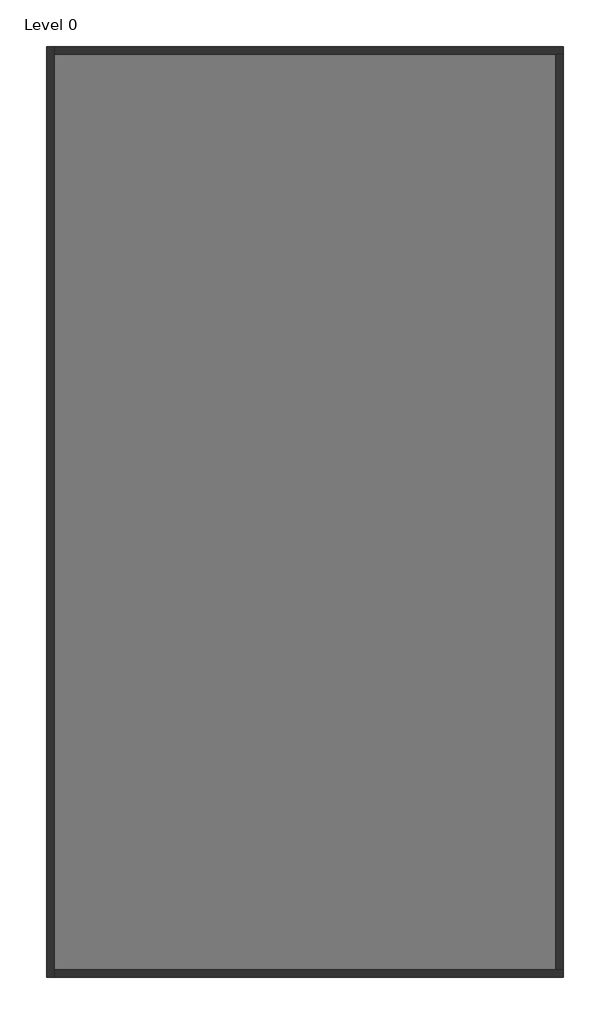
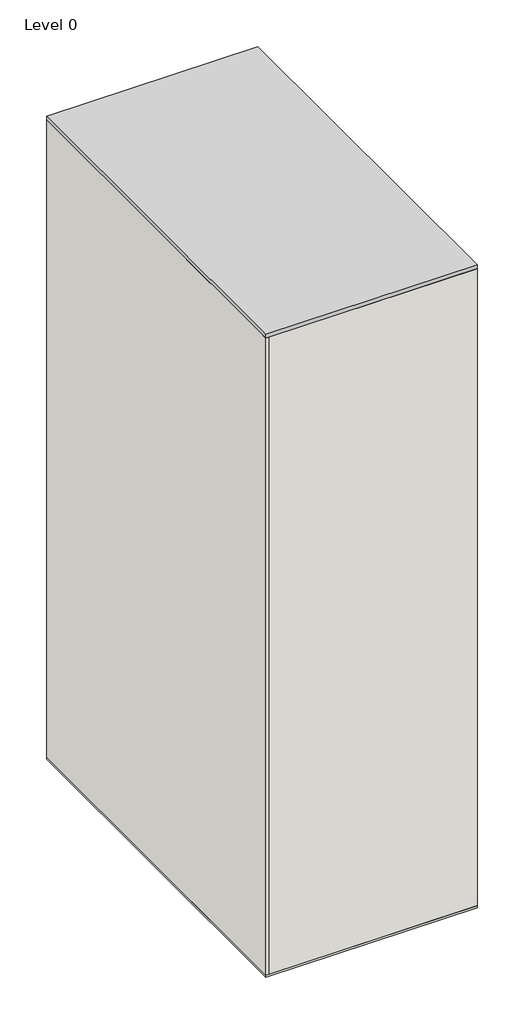
# One storey: 4 walls, 1 proxy, 1 slab.
"""IFC4 building model written with IfcOpenShell, lengths in millimetres."""

from ifc_helpers import new_model, si_unit, frame, origin, origin_with_axes, place, context, project, spatial, polyline, outline, extrude, faceted_brep, element, save

model = new_model("IFC4")

# Units and contexts
model_context = context("Model", 3, world=origin())
ifc_project = project(units=[si_unit("LENGTHUNIT", "METRE", prefix="MILLI")], contexts=[model_context])

# Site, building, storey
site = spatial("IfcSite", under=ifc_project)
building = spatial("IfcBuilding", under=site)
storey = spatial("IfcBuildingStorey", under=building, Name="Level 0", Elevation=100.0)

# Proxy
placement = place(None, origin())
element("IfcBuildingElementProxy", 1, Name="LowUrbanDensityBuilding : LowUrbanDensityBuilding", ObjectType="LowUrbanDensityBuilding : LowUrbanDensityBuilding", at=placement, inside=storey, context=model_context, shape_type="SweptSolid", body=[
    extrude(outline(polyline([(7325.2659446, 3676.2074539), (7325.2659446, -14323.7925461), (-2674.7340554, -14323.7925461), (-2674.7340554, 3676.2074539), (7325.2659446, 3676.2074539)])), origin_with_axes(), (0.0, 0.0, 1.0), 32200.0),
])

# Slab
element("IfcSlab", 2, ObjectType="Floor-Concrete_100Con", at=placement, inside=storey, context=model_context, shape_type="SweptSolid", body=[
    extrude(outline(polyline([(7325.2659446, 3676.2074539), (7325.2659446, -14323.7925461), (-2674.7340554, -14323.7925461), (-2674.7340554, 3676.2074539), (7325.2659446, 3676.2074539)])), origin_with_axes(), (0.0, 0.0, 1.0), 100.0),
])

# Walls
element("IfcWall", 3, ObjectType="Wall-Ext_25Rdr-100Blk-19P", at=placement, inside=storey, context=model_context, shape_type="Brep", body=[
    faceted_brep([(-2674.7340554, 3676.2074539, 100.0), (-2674.7340554, -14323.7925461, 100.0), (-2674.7340554, -14323.7925461, 32000.0), (-2674.7340554, 3676.2074539, 32000.0), (-2530.4340554, 3676.2074539, 100.0), (-2530.4340554, 3676.2074539, 32000.0), (-2530.4340554, 3531.9074539, 32000.0), (-2530.4340554, -14179.4925461, 32000.0), (-2530.4340554, -14323.7925461, 32000.0), (-2530.4340554, -14323.7925461, 100.0), (-2530.4340554, -14179.4925461, 100.0), (-2530.4340554, 3531.9074539, 100.0)], [[[0, 1, 2, 3]], [[4, 5, 6, 7, 8, 9, 10, 11]], [[1, 0, 4, 11, 10, 9]], [[3, 2, 8, 7, 6, 5]], [[2, 1, 9, 8]], [[0, 3, 5, 4]]]),
])
element("IfcWall", 4, ObjectType="Wall-Ext_25Rdr-100Blk-19P", at=placement, inside=storey, context=model_context, shape_type="Brep", body=[
    faceted_brep([(-2530.4340554, -14323.7925461, 100.0), (7325.2659446, -14323.7925461, 100.0), (7325.2659446, -14323.7925461, 32000.0), (-2530.4340554, -14323.7925461, 32000.0), (-2530.4340554, -14179.4925461, 100.0), (-2530.4340554, -14179.4925461, 32000.0), (7180.9659446, -14179.4925461, 32000.0), (7325.2659446, -14179.4925461, 32000.0), (7325.2659446, -14179.4925461, 100.0), (7180.9659446, -14179.4925461, 100.0)], [[[0, 1, 2, 3]], [[4, 5, 6, 7, 8, 9]], [[1, 0, 4, 9, 8]], [[3, 2, 7, 6, 5]], [[0, 3, 5, 4]], [[2, 1, 8, 7]]]),
])
element("IfcWall", 5, ObjectType="Wall-Ext_25Rdr-100Blk-19P", at=placement, inside=storey, context=model_context, shape_type="Brep", body=[
    faceted_brep([(7325.2659446, 3676.2074539, 100.0), (-2530.4340554, 3676.2074539, 100.0), (-2530.4340554, 3676.2074539, 32000.0), (7325.2659446, 3676.2074539, 32000.0), (7325.2659446, 3531.9074539, 100.0), (7325.2659446, 3531.9074539, 32000.0), (7180.9659446, 3531.9074539, 32000.0), (-2530.4340554, 3531.9074539, 32000.0), (-2530.4340554, 3531.9074539, 100.0), (7180.9659446, 3531.9074539, 100.0)], [[[0, 1, 2, 3]], [[4, 5, 6, 7, 8, 9]], [[1, 0, 4, 9, 8]], [[3, 2, 7, 6, 5]], [[2, 1, 8, 7]], [[0, 3, 5, 4]]]),
])
element("IfcWall", 6, ObjectType="Wall-Ext_25Rdr-100Blk-19P", at=placement, inside=storey, context=model_context, shape_type="SweptSolid", body=[
    extrude(outline(polyline([(7325.2659446, 3531.9074539), (7325.2659446, -14179.4925461), (7180.9659446, -14179.4925461), (7180.9659446, 3531.9074539), (7325.2659446, 3531.9074539)])), frame((0.0, 0.0, 100.0), z_axis=(0.0, 0.0, 1.0), x_axis=(1.0, 0.0, 0.0)), (0.0, 0.0, 1.0), 31900.0),
])

save(model, "model.ifc")

# Revit data of these elements
# Project information
#   Project Issue Date = "Issue Date"
#   Project Status = "Project Status"
#   Client Name = "Owner"
#   Project Address = "Enter address here"
#   Project Name = "Project Name"
#   Project Number = "Project Number"
# Type "Floor-Concrete_100Con"
#   Keynote = "E60/130"
#   Function = 0
#   Layers, outside or top first: 100 mm "Concrete" (function 1)
# Type "Wall-Ext_25Rdr-100Blk-19P"
#   Keynote = "F10"
#   Layers, outside or top first: 25.3 mm "Render, Beige, Smooth" (function 5); 100 mm "Concrete Masonry Units _Low Density" (function 1); 19 mm "Plaster" (function 5)
# Element 1 (IfcBuildingElementProxy, "LowUrbanDensityBuilding : LowUrbanDensityBuilding")
#   Phase Created = New Construction
#   Materials on its faces: "Default Form"
# Element 2 (IfcSlab, "Floor-Concrete_100Con")
#   Height Offset From Level = 0 mm
#   Phase Created = New Construction
#   Materials on its faces: "Concrete"
# Element 3 (IfcWall, "Wall-Ext_25Rdr-100Blk-19P")
#   Top Offset = 0 mm
#   Base Offset = 0 mm
#   wall height = 31900 mm
#   Phase Created = New Construction
#   Base Constraint = Level 0
#   Top Constraint = Level 8
#   Materials on its faces: "Render, Beige, Smooth", "Default Wall", "Plaster"
# Elements 4, 5, 6 (IfcWall, "Wall-Ext_25Rdr-100Blk-19P")
#   Top Offset = 0 mm
#   Base Offset = 0 mm
#   wall height = 31900 mm
#   Phase Created = New Construction
#   Base Constraint = Level 0
#   Top Constraint = Level 8
#   Materials on its faces: "Default Wall", "Render, Beige, Smooth", "Plaster"
# Materials
#   "Concrete": class "Concrete", colour RGB 120 120 120, transparency 0, Description = "Portland Cement Concrete", Cost = 0
#   "Render, Beige, Smooth": class "Generic", colour RGB 213 198 180, transparency 0, Description = "physical material", Cost = 0
#   "Concrete Masonry Units _Low Density": class "Masonry", colour RGB 181 181 181, transparency 0, Description = "Concrete masonry units", Cost = 0
#   "Plaster": class "Generic", colour RGB 249 249 249, transparency 0, Description = "Plaster", Cost = 0
#   "Default Form": class "Generic", colour RGB 185 189 196, transparency 0.5, Cost = 0
#   "Default Wall": class "Miscellaneous", colour RGB 128 128 128, transparency 0, Comments = "Rendering appearance not upgraded Rendering appearance not upgraded ", Cost = 0
